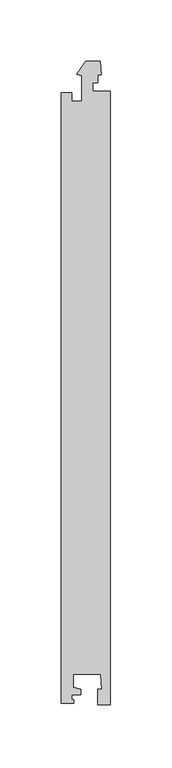
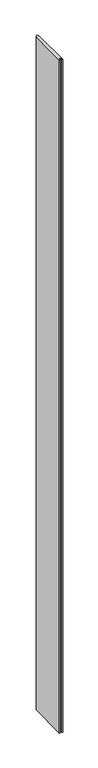
"""IFC4 building model written with IfcOpenShell, lengths in millimetres: proxy geometry, Generic Models 5:Generic Models 5:321804:Generic Models 5:321804 : Generic Models 5:Generic Models 5:321804:37 : Generic Models 5:Generic Models 5:321804:Generic Models 5:321804 : Generic Models 5:Generic Models 5:321804:300761."""

from ifc_helpers import new_model, si_unit, frame, origin, place, context, project, spatial, polyline, outline, extrude, source, transform, mapped, element, save


def generic_models_7dd7d513(model_context):
    return source(origin(), model_context, "Body", "SweptSolid", [
        extrude(outline(polyline([(667625.2338797, -490910.833465), (667631.7338797, -490912.5751348), (667631.7338797, -490917.0251348), (667624.2338797, -490917.0251348), (667624.2338797, -490920.9751348), (667625.7338797, -490920.9751348), (667625.7338797, -490923.9751348), (667615.7338797, -490923.9751348), (667615.7338797, -490426.4751348), (667624.2338797, -490426.4751348), (667624.2338797, -490433.4251348), (667632.2338797, -490433.4251348), (667632.2338797, -490412.7091094), (667628.3059983, -490411.6566367), (667635.4133634, -490400.9751348), (667647.2715044, -490400.9751348), (667648.2338797, -490411.9751348), (667645.5338797, -490411.9751348), (667645.5338797, -490418.6001348), (667641.2338797, -490418.6001348), (667641.2338797, -490425.2251348), (667655.7338797, -490425.2251348), (667655.7338797, -490925.2251348), (667645.5338797, -490925.2251348), (667645.5338797, -490912.4751348), (667648.779534, -490912.4751348), (667647.72967, -490900.4751348), (667625.2338797, -490900.4751348), (667625.2338797, -490910.833465)])), frame((0.0, 0.0, -5.8417589), z_axis=(0.0, 0.0, 1.0), x_axis=(1.0, 0.0, 0.0)), (0.0, 0.0, 1.0), 8779.7126309),
    ])


if __name__ == "__main__":
    model = new_model("IFC4")
    model_context = context("Model", 3, world=origin())
    ifc_project = project(units=[si_unit("LENGTHUNIT", "METRE", prefix="MILLI")], contexts=[model_context])
    site = spatial("IfcSite", under=ifc_project)
    building = spatial("IfcBuilding", under=site)
    placement = place(None, origin())
    generic_models_shape = generic_models_7dd7d513(model_context)
    element("IfcBuildingElementProxy", 1, Name="Generic Models 5:Generic Models 5:321804:Generic Models 5:321804 : Generic Models 5:Generic Models 5:321804:37 : Generic Models 5:Generic Models 5:321804:Generic Models 5:321804 : Generic Models 5:Generic Models 5:321804:300761", ObjectType="Generic Models 5:Generic Models 5:321804:Generic Models 5:321804 : Generic Models 5:Generic Models 5:321804:37 : Generic Models 5:Generic Models 5:321804:Generic Models 5:321804 : Generic Models 5:Generic Models 5:321804:300761", at=placement, inside=building, context=model_context, shape_type="MappedRepresentation", body=[
        mapped(generic_models_shape, transform((0.0, 0.0, 0.0), x_axis=(1.0, 0.0, 0.0), y_axis=(0.0, 1.0, 0.0), z_axis=(0.0, 0.0, 1.0))),
    ])
    save(model, "model.ifc")

# Revit data of these elements
# Type "Generic Models 5:Generic Models 5:321804:Generic Models 5:321804 : Generic Models 5:Generic Models 5:321804:37 : Generic Models 5:Generic Models 5:321804:Generic Models 5:321804 : Generic Models 5:Generic Models 5:321804:300761"
#   NameOverride = "Generic Models 5:Generic Models 5:321804:Generic Models 5:321804 : Generic Models 5:Generic Models 5:321804:300761"
#   ObjectTypeOverride = "Generic Models 5:321804 : Generic Models 5:Generic Models 5:321804"
#   Reference = "Generic Models 5"
#   Tag = "300761"
# Element 1 (IfcBuildingElementProxy, "Generic Models 5:Generic Models 5:321804:Generic Models 5:321804 : Generic Models 5:Generic Models 5:321804:37 : Generic Models 5:Generic Models 5:321804:Generic Models 5:321804 : Generic Models 5:Generic Models 5:321804:300761")
#   Materials on its faces: "POLYCARBONATE PANEL - ARCOPLUS 547"
# Materials
#   "POLYCARBONATE PANEL - ARCOPLUS 547": class "Unassigned", colour RGB 202 225 249, transparency 0.45, Cost = 0
